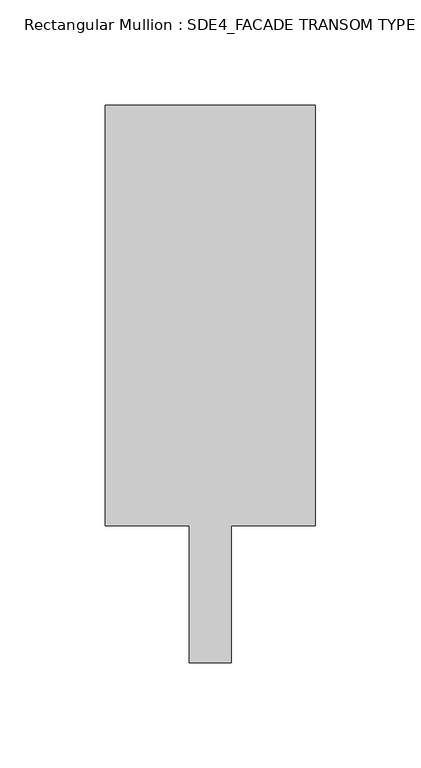
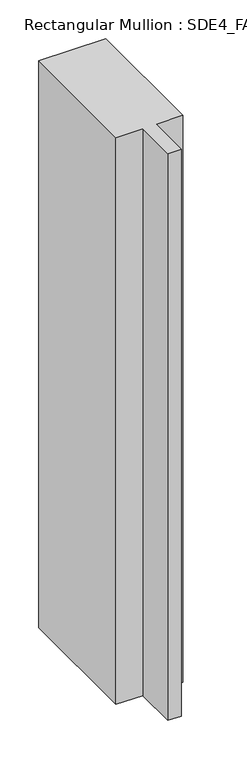
"""IFC4 building model written with IfcOpenShell, lengths in millimetres: member geometry, Rectangular Mullion : SDE4_FACADE TRANSOM TYPE 2."""

from ifc_helpers import new_model, si_unit, frame, origin, place, context, project, spatial, polyline, outline, extrude, source, transform, mapped, element, save


def rectangular_mullion_sde4_facade_transom_type_2_e5ccb255(model_context):
    return source(origin(), model_context, "Body", "SweptSolid", [
        extrude(outline(polyline([(50.0, 132.5), (50.0, -67.5), (10.0, -67.5), (10.0, -132.5), (-10.0, -132.5), (-10.0, -67.5), (-50.0, -67.5), (-50.0, 132.5), (50.0, 132.5)])), frame((0.0, 0.0, -895.25), z_axis=(0.0, 0.0, 1.0), x_axis=(1.0, 0.0, 0.0)), (0.0, 0.0, 1.0), 895.25),
    ])


if __name__ == "__main__":
    model = new_model("IFC4")
    model_context = context("Model", 3, world=origin())
    ifc_project = project(units=[si_unit("LENGTHUNIT", "METRE", prefix="MILLI")], contexts=[model_context])
    site = spatial("IfcSite", under=ifc_project)
    building = spatial("IfcBuilding", under=site)
    placement = place(None, origin())
    rectangular_mullion_sde4_facade_transom_type_2_shape = rectangular_mullion_sde4_facade_transom_type_2_e5ccb255(model_context)
    element("IfcMember", 1, ObjectType="Rectangular Mullion : SDE4_FACADE TRANSOM TYPE 2", at=placement, inside=building, context=model_context, shape_type="MappedRepresentation", body=[
        mapped(rectangular_mullion_sde4_facade_transom_type_2_shape, transform((0.0, 0.0, 0.0), x_axis=(1.0, 0.0, 0.0), y_axis=(0.0, 1.0, 0.0), z_axis=(0.0, 0.0, 1.0))),
    ])
    save(model, "model.ifc")

# Revit data of these elements
# Type "Rectangular Mullion : SDE4_FACADE TRANSOM TYPE 2"
#   built-in parameter 1007322 = 0.869423 (stored number, unit not read)
#   built-in parameter 1007321 = 0.164042 (stored number, unit not read)
#   built-in parameter 1007320 = 0.164042 (stored number, unit not read)
